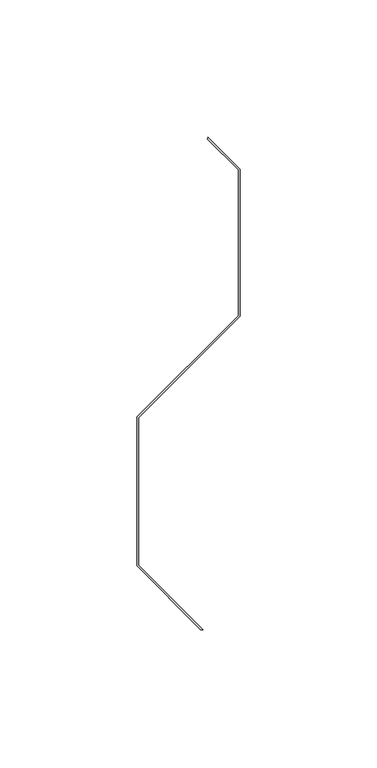
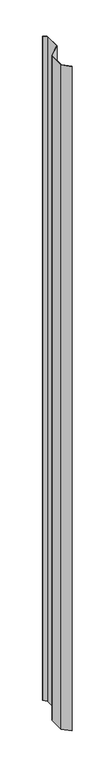
"""IFC4 building model written with IfcOpenShell, lengths in millimetres: proxy geometry, MBCI 7.2-V Panel10 : MBCI 7.2-V Panel-1."""

from ifc_helpers import new_model, si_unit, frame, origin, place, context, project, spatial, polyline, outline, extrude, source, transform, mapped, element, save


def generic_models_064e3d49(model_context):
    return source(origin(), model_context, "Body", "SweptSolid", [
        extrude(outline(polyline([(587365.2695864, -532763.3383203), (587328.3744989, -532800.2334078), (587328.3744989, -532854.0208986), (587351.8199844, -532877.4663841), (587350.9780854, -532877.4663841), (587327.7791864, -532854.2674851), (587327.7791864, -532799.9868213), (587364.6742739, -532763.0917338), (587364.6742739, -532710.0036068), (587353.54384, -532698.8731729), (587353.5988637, -532698.0862976), (587365.2695864, -532709.7570203), (587365.2695864, -532763.3383203)])), frame((0.0, 0.0, 51.59375), z_axis=(0.0, 0.0, 1.0), x_axis=(1.0, 0.0, 0.0)), (0.0, 0.0, 1.0), 2386.80625),
    ])


if __name__ == "__main__":
    model = new_model("IFC4")
    model_context = context("Model", 3, world=origin())
    ifc_project = project(units=[si_unit("LENGTHUNIT", "METRE", prefix="MILLI")], contexts=[model_context])
    site = spatial("IfcSite", under=ifc_project)
    building = spatial("IfcBuilding", under=site)
    placement = place(None, origin())
    generic_models_shape = generic_models_064e3d49(model_context)
    element("IfcBuildingElementProxy", 1, Name="MBCI 7.2-V Panel10 : MBCI 7.2-V Panel-1", ObjectType="MBCI 7.2-V Panel10 : MBCI 7.2-V Panel-1", at=placement, inside=building, context=model_context, shape_type="MappedRepresentation", body=[
        mapped(generic_models_shape, transform((0.0, 0.0, 0.0), x_axis=(1.0, 0.0, 0.0), y_axis=(0.0, 1.0, 0.0), z_axis=(0.0, 0.0, 1.0))),
    ])
    save(model, "model.ifc")

# Revit data of these elements
# Element 1 (IfcBuildingElementProxy, "MBCI 7.2-V Panel10 : MBCI 7.2-V Panel-1")
#   Materials on its faces: "MTL PANEL"
# Materials
#   "MTL PANEL": class "Generic", colour RGB 239 242 240, transparency 0, Cost = 0
